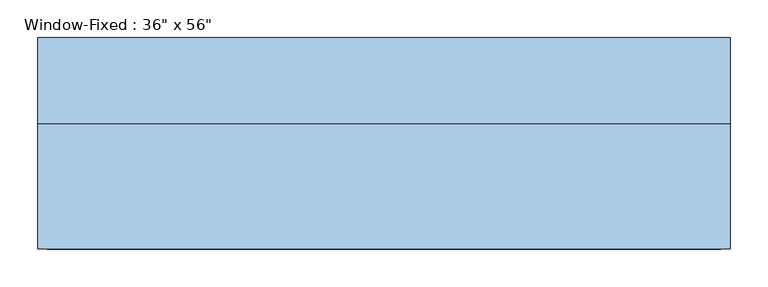
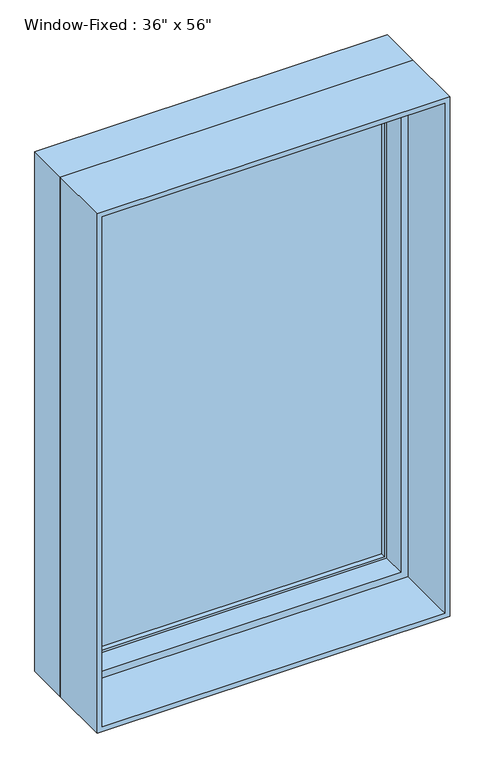
"""IFC4 building model written with IfcOpenShell, lengths in millimetres: window geometry."""

from ifc_helpers import new_model, si_unit, frame, origin, place, context, project, spatial, polyline, outline, extrude, faceted_brep, source, transform, mapped, element, save


def window_fe4c84aa(model_context):
    return source(origin(), model_context, "Body", "SolidModel", [
        extrude(outline(polyline([(419.1, 104.775), (419.1, 98.425), (-419.1, 98.425), (-419.1, 104.775), (419.1, 104.775)])), frame((0.0, 0.0, 952.5), z_axis=(0.0, 0.0, 1.0), x_axis=(1.0, 0.0, 0.0)), (0.0, 0.0, 1.0), 1346.2),
        extrude(outline(polyline([(-419.1, 85.725), (-419.1, 92.075), (419.1, 92.075), (419.1, 85.725), (-419.1, 85.725)])), frame((0.0, 0.0, 952.5), z_axis=(0.0, 0.0, 1.0), x_axis=(1.0, 0.0, 0.0)), (0.0, 0.0, 1.0), 1346.2),
        extrude(outline(polyline([(927.1, 444.5), (2324.1, 444.5), (2324.1, -444.5), (927.1, -444.5), (927.1, 444.5)]), holes=[polyline([(952.5, -419.1), (2298.7, -419.1), (2298.7, 419.1), (952.5, 419.1), (952.5, -419.1)])]), frame((0.0, 73.025, 0.0), z_axis=(0.0, 1.0, 0.0), x_axis=(0.0, 0.0, 1.0)), (0.0, 0.0, 1.0), 44.45),
        extrude(outline(polyline([(2336.8, -457.2), (914.4, -457.2), (914.4, 457.2), (2336.8, 457.2), (2336.8, -457.2)]), holes=[polyline([(2324.1, 444.5), (927.1, 444.5), (927.1, -444.5), (2324.1, -444.5), (2324.1, 444.5)])]), frame((0.0, -155.575, 0.0), z_axis=(0.0, 1.0, 0.0), x_axis=(0.0, 0.0, 1.0)), (0.0, 0.0, 1.0), 165.1),
        faceted_brep([(457.2, 9.525, 2336.8), (457.2, 123.825, 2336.8), (-457.2, 123.825, 2336.8), (-457.2, 9.525, 2336.8), (-457.2, 123.825, 914.4), (-457.2, 9.525, 914.4), (457.2, 123.825, 914.4), (457.2, 9.525, 914.4), (425.45, 9.525, 2305.05), (425.45, 9.525, 946.15), (-425.45, 9.525, 946.15), (-425.45, 9.525, 2305.05), (-444.5, 123.825, 2324.1), (-444.5, 123.825, 927.1), (444.5, 123.825, 927.1), (444.5, 123.825, 2324.1), (425.45, 73.025, 2305.05), (-425.45, 73.025, 2305.05), (444.5, 73.025, 2324.1), (-444.5, 73.025, 2324.1), (-425.45, 73.025, 946.15), (-444.5, 73.025, 927.1), (425.45, 73.025, 946.15), (444.5, 73.025, 927.1)], [[[0, 1, 2, 3]], [[3, 2, 4, 5]], [[5, 4, 6, 7]], [[3, 5, 7, 0], [8, 9, 10, 11]], [[7, 6, 1, 0]], [[1, 6, 4, 2], [12, 13, 14, 15]], [[16, 8, 11, 17]], [[15, 18, 19, 12]], [[17, 11, 10, 20]], [[12, 19, 21, 13]], [[20, 10, 9, 22]], [[13, 21, 23, 14]], [[22, 9, 8, 16]], [[18, 23, 21, 19], [17, 20, 22, 16]], [[14, 23, 18, 15]]]),
    ])


if __name__ == "__main__":
    model = new_model("IFC4")
    model_context = context("Model", 3, world=origin())
    ifc_project = project(units=[si_unit("LENGTHUNIT", "METRE", prefix="MILLI")], contexts=[model_context])
    site = spatial("IfcSite", under=ifc_project)
    building = spatial("IfcBuilding", under=site)
    placement = place(None, origin())
    window_shape = window_fe4c84aa(model_context)
    element("IfcWindow", 1, ObjectType="Window-Fixed : 36\" x 56\"", at=placement, inside=building, context=model_context, shape_type="MappedRepresentation", body=[
        mapped(window_shape, transform((0.0, 0.0, 0.0), x_axis=(1.0, 0.0, 0.0), y_axis=(0.0, 1.0, 0.0), z_axis=(0.0, 0.0, 1.0))),
    ])
    save(model, "model.ifc")

# Revit data of these elements
# Type "Window-Fixed : 36\" x 56\""
#   Type Mark = "22"
#   Fire Rating = "0.5h"
#   Assembly Code = "B2020100"
#   Analytic Construction = "Double glazing - domestic"
#   Window Inset [instance default] = 0' - 0"
#   Wall Thickness [instance default] = 0' - 6"
#   Visual Light Transmittance = 0.81
#   Thermal Resistance (R) = 1.8146 (h·ft²·°F)/BTU
#   Solar Heat Gain Coefficient = 0.76
#   Rough Width = 3' - 0 1/2"
#   Rough Height = 4' - 8 1/2"
#   Interior Wall Closure [instance default] = 0' - 2 1/4"
#   Height = 4' - 8"
#   Heat Transfer Coefficient (U) = 0.5511 BTU/(h·ft²·°F)
#   Frame Extension [instance default] = 0' - 0 1/4"
#   Exterior Wall Closure [instance default] = 0' - 1 1/4"
#   Extension Jamb [instance default] = 0' - 2 1/4"
#   Default Sill Height = 3' - 0"
#   Width = 3' - 0"
#   Muntin Visibility = yes
#   Interior Trim Visibility [instance default] = yes
#   Exterior Trim Visibility [instance default] = yes
#   Extension Jamb Visibility [instance default] = yes
#   Muntin Pattern = Muntin Pattern_2x2 : Muntin Pattern_2x2
#   Interior Trim Material = Wood - Stained
#   Interior Trim = Trim-Window-Interior-Flat : Picture Frame
#   Interior Frame Material = Wood - Stained
#   Glass Panel Material = Glass
#   Exterior Trim Material = Clad - White
#   Exterior Trim = Trim-Window-Exterior-Flat : with Sill
#   Exterior Frame Material = Clad - White
#   Wall Closure = (empty or 0)
# Element 1 (IfcWindow, "Window-Fixed : 36\" x 56\"")
#   Window Inset = 0' - 2"
#   Wall Thickness = 1' - 0 1/4"
#   Exterior Wall Closure = 0' - 5 1/2"
#   Extension Jamb = 0' - 6 1/2"
#   Exterior Trim Visibility = no
#   Materials on its faces: "Wood - Stained", "Glass", "Clad - White"
# Materials
#   "Wood - Stained": class "Wood", colour RGB 224 178 126, transparency 0, Cost = 0
#   "Glass": class "Glass", colour RGB 0 128 192, transparency 0.75, Description = "Soda Lime Glass", Cost = 0
#   "Clad - White": class "Wood", colour RGB 242 242 238, transparency 0, Cost = 0
